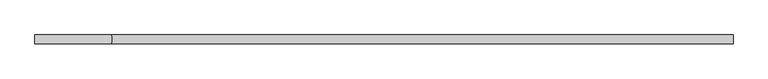
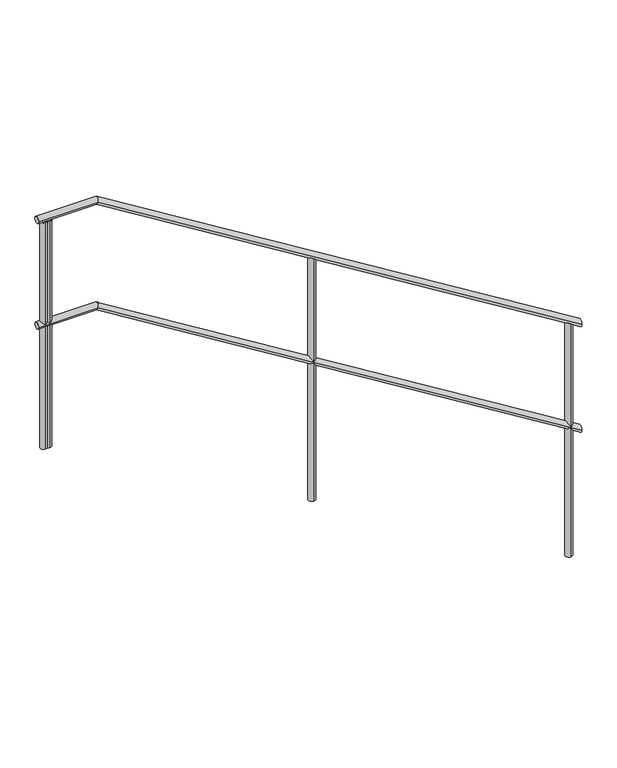
"""IFC4 building model written with IfcOpenShell, lengths in millimetres: railing geometry."""

from ifc_helpers import new_model, si_unit, point, frame, frame_2d, origin, place, context, project, spatial, circle_curve, ellipse_curve, trimmed, segment, composite_curve, outline, extrude, source, transform, mapped, element, save
from ifc_brep_helpers import plane_surface, cylinder_surface, advanced_brep


def railing_0facc66a(model_context):
    return source(origin(), model_context, "Body", "SolidModel", [
        advanced_brep(
        [(33992.1378478, 64692.0208589, -450.9609787), (33992.1378478, 64662.0208589, -450.9609787), (31827.8810623, 64692.0208589, 885.0), (31827.8810623, 64662.0208589, 885.0), (31562.1378478, 64692.0208589, 885.0), (31562.1378478, 64662.0208589, 885.0)],
        [
            (0, 1, ellipse_curve(frame((33992.1378478, 64677.0208589, -450.9609787), z_axis=(1.0, 0.0, 0.0), x_axis=(0.0, 0.0, -1.0)), 17.6276454, 15.0)),
            (1, 0, ellipse_curve(frame((33992.1378478, 64677.0208589, -450.9609787), z_axis=(1.0, 0.0, 0.0), x_axis=(0.0, 0.0, -1.0)), 17.6276454, 15.0)),
            (0, 2),
            (2, 3, ellipse_curve(frame((31827.8810623, 64677.0208589, 885.0), z_axis=(0.9620125025549408, 0.0, -0.2730053935877092), x_axis=(-0.2730053935877086, 0.0, -0.9620125025549411)), 15.5923129, 15.0)),
            (3, 1),
            (3, 2, ellipse_curve(frame((31827.8810623, 64677.0208589, 885.0), z_axis=(0.9620125025549408, 0.0, -0.2730053935877092), x_axis=(-0.2730053935877086, 0.0, -0.9620125025549411)), 15.5923129, 15.0)),
            (4, 5, circle_curve(frame((31562.1378478, 64677.0208589, 885.0), z_axis=(-1.0, 0.0, 0.0), x_axis=(0.0, -1.0, 0.0)), 15.0)),
            (5, 4, circle_curve(frame((31562.1378478, 64677.0208589, 885.0), z_axis=(-1.0, 0.0, 0.0), x_axis=(0.0, -1.0, 0.0)), 15.0)),
            (2, 4),
            (5, 3),
        ],
        [
            plane_surface(frame((33992.1378478, 64677.0208589, -433.3333333), z_axis=(1.0, 0.0, 0.0), x_axis=(0.0, -1.0, 0.0))),
            cylinder_surface(frame((33984.2588097, 64677.0208589, -446.097375), z_axis=(0.8509361101440399, 0.0, -0.5252692037926175), x_axis=(0.0, -1.0, 0.0)), 15.0),
            plane_surface(frame((31562.1378478, 64677.0208589, 900.0), z_axis=(-1.0, 0.0, 0.0), x_axis=(0.0, -1.0, 0.0))),
            cylinder_surface(frame((31832.1378478, 64677.0208589, 885.0), z_axis=(1.0, 0.0, 0.0), x_axis=(0.0, -1.0, 0.0)), 15.0),
        ],
        [
            (0, [[1, 2]]),
            (1, [[-1, 3, 4, 5]]),
            (1, [[-2, -5, 6, -3]]),
            (2, [[7, 8]]),
            (3, [[-4, 9, -8, 10]]),
            (3, [[-6, -10, -7, -9]]),
        ],
    ),
        advanced_brep(
        [(33992.1378478, 64692.0208589, 49.0390213), (33992.1378478, 64662.0208589, 49.0390213), (31827.8810623, 64692.0208589, 1385.0), (31827.8810623, 64662.0208589, 1385.0), (31562.1378478, 64692.0208589, 1385.0), (31562.1378478, 64662.0208589, 1385.0)],
        [
            (0, 1, ellipse_curve(frame((33992.1378478, 64677.0208589, 49.0390213), z_axis=(1.0, 0.0, 0.0), x_axis=(0.0, 0.0, -1.0)), 17.6276454, 15.0)),
            (1, 0, ellipse_curve(frame((33992.1378478, 64677.0208589, 49.0390213), z_axis=(1.0, 0.0, 0.0), x_axis=(0.0, 0.0, -1.0)), 17.6276454, 15.0)),
            (0, 2),
            (2, 3, ellipse_curve(frame((31827.8810623, 64677.0208589, 1385.0), z_axis=(0.9620125025549408, 0.0, -0.2730053935877092), x_axis=(-0.2730053935877086, 0.0, -0.9620125025549411)), 15.5923129, 15.0)),
            (3, 1),
            (3, 2, ellipse_curve(frame((31827.8810623, 64677.0208589, 1385.0), z_axis=(0.9620125025549408, 0.0, -0.2730053935877092), x_axis=(-0.2730053935877086, 0.0, -0.9620125025549411)), 15.5923129, 15.0)),
            (4, 5, circle_curve(frame((31562.1378478, 64677.0208589, 1385.0), z_axis=(-1.0, 0.0, 0.0), x_axis=(0.0, -1.0, 0.0)), 15.0)),
            (5, 4, circle_curve(frame((31562.1378478, 64677.0208589, 1385.0), z_axis=(-1.0, 0.0, 0.0), x_axis=(0.0, -1.0, 0.0)), 15.0)),
            (2, 4),
            (5, 3),
        ],
        [
            plane_surface(frame((33992.1378478, 64677.0208589, 66.6666667), z_axis=(1.0, 0.0, 0.0), x_axis=(0.0, -1.0, 0.0))),
            cylinder_surface(frame((33984.2588097, 64677.0208589, 53.902625), z_axis=(0.8509361101440399, 0.0, -0.5252692037926175), x_axis=(0.0, -1.0, 0.0)), 15.0),
            plane_surface(frame((31562.1378478, 64677.0208589, 1400.0), z_axis=(-1.0, 0.0, 0.0), x_axis=(0.0, -1.0, 0.0))),
            cylinder_surface(frame((31832.1378478, 64677.0208589, 1385.0), z_axis=(1.0, 0.0, 0.0), x_axis=(0.0, -1.0, 0.0)), 15.0),
        ],
        [
            (0, [[1, 2]]),
            (1, [[-1, 3, 4, 5]]),
            (1, [[-2, -5, 6, -3]]),
            (2, [[7, 8]]),
            (3, [[-4, 9, -8, 10]]),
            (3, [[-6, -10, -7, -9]]),
        ],
    ),
        extrude(outline(composite_curve([segment(trimmed(circle_curve(frame_2d((31592.1378478, 64677.0208589)), 15.0), [point((31592.1378478, 64692.0208589))], [point((31592.1378478, 64662.0208589))], False, "CARTESIAN"), True, "CONTINUOUS"), segment(trimmed(circle_curve(frame_2d((31592.1378478, 64677.0208589)), 15.0), [point((31592.1378478, 64662.0208589))], [point((31592.1378478, 64692.0208589))], False, "CARTESIAN"), True, "CONTINUOUS")], self_intersect=False)), frame((0.0, 0.0, 300.0), z_axis=(0.0, 0.0, 1.0), x_axis=(1.0, 0.0, 0.0)), (0.0, 0.0, 1.0), 1070.0),
        advanced_brep(
        [(32792.1378478, 64662.0208589, 777.4074074), (32792.1378478, 64692.0208589, 777.4074074), (32792.1378478, 64692.0208589, -366.6666667), (32792.1378478, 64662.0208589, -366.6666667)],
        [
            (0, 1, ellipse_curve(frame((32792.1378478, 64677.0208589, 777.4074074), z_axis=(-0.5252692037926167, 0.0, -0.8509361101440406), x_axis=(-0.8509361101440406, 0.0, 0.5252692037926162)), 17.6276454, 15.0)),
            (1, 2),
            (2, 3, circle_curve(frame((32792.1378478, 64677.0208589, -366.6666667), z_axis=(0.0, 0.0, 1.0), x_axis=(0.0, 1.0, 0.0)), 15.0)),
            (3, 0),
            (3, 2, circle_curve(frame((32792.1378478, 64677.0208589, -366.6666667), z_axis=(0.0, 0.0, 1.0), x_axis=(0.0, 1.0, 0.0)), 15.0)),
            (1, 0, ellipse_curve(frame((32792.1378478, 64677.0208589, 777.4074074), z_axis=(-0.5252692037926167, 0.0, -0.8509361101440406), x_axis=(-0.8509361101440406, 0.0, 0.5252692037926162)), 17.6276454, 15.0)),
        ],
        [
            cylinder_surface(frame((32792.1378478, 64677.0208589, -466.6666667), z_axis=(0.0, 0.0, 1.0), x_axis=(0.0, 1.0, 0.0)), 15.0),
            plane_surface(frame((32767.1378478, 64702.0208589, 792.8395062), z_axis=(0.5252692037926167, 0.0, 0.8509361101440406), x_axis=(0.0, -1.0, 0.0))),
            plane_surface(frame((32817.1378478, 64702.0208589, -366.6666667), z_axis=(0.0, 0.0, -1.0), x_axis=(0.0, -1.0, 0.0))),
        ],
        [
            (0, [[1, 2, 3, 4]]),
            (0, [[5, -2, 6, -4]]),
            (1, [[-6, -1]]),
            (2, [[-5, -3]]),
        ],
    ),
        extrude(outline(composite_curve([segment(trimmed(circle_curve(frame_2d((31612.1378478, 64677.0208589)), 15.0), [point((31612.1378478, 64692.0208589))], [point((31612.1378478, 64662.0208589))], False, "CARTESIAN"), True, "CONTINUOUS"), segment(trimmed(circle_curve(frame_2d((31612.1378478, 64677.0208589)), 15.0), [point((31612.1378478, 64662.0208589))], [point((31612.1378478, 64692.0208589))], False, "CARTESIAN"), True, "CONTINUOUS")], self_intersect=False)), frame((0.0, 0.0, 300.0), z_axis=(0.0, 0.0, 1.0), x_axis=(1.0, 0.0, 0.0)), (0.0, 0.0, 1.0), 1070.0),
        advanced_brep(
        [(33942.1378478, 64662.0208589, 67.5308642), (33942.1378478, 64692.0208589, 67.5308642), (33942.1378478, 64692.0208589, -1033.3333333), (33942.1378478, 64662.0208589, -1033.3333333)],
        [
            (0, 1, ellipse_curve(frame((33942.1378478, 64677.0208589, 67.5308642), z_axis=(-0.5252692037926167, 0.0, -0.8509361101440406), x_axis=(-0.8509361101440406, 0.0, 0.5252692037926162)), 17.6276454, 15.0)),
            (1, 2),
            (2, 3, circle_curve(frame((33942.1378478, 64677.0208589, -1033.3333333), z_axis=(0.0, 0.0, 1.0), x_axis=(0.0, 1.0, 0.0)), 15.0)),
            (3, 0),
            (3, 2, circle_curve(frame((33942.1378478, 64677.0208589, -1033.3333333), z_axis=(0.0, 0.0, 1.0), x_axis=(0.0, 1.0, 0.0)), 15.0)),
            (1, 0, ellipse_curve(frame((33942.1378478, 64677.0208589, 67.5308642), z_axis=(-0.5252692037926167, 0.0, -0.8509361101440406), x_axis=(-0.8509361101440406, 0.0, 0.5252692037926162)), 17.6276454, 15.0)),
        ],
        [
            cylinder_surface(frame((33942.1378478, 64677.0208589, -1133.3333333), z_axis=(0.0, 0.0, 1.0), x_axis=(0.0, 1.0, 0.0)), 15.0),
            plane_surface(frame((33917.1378478, 64702.0208589, 82.962963), z_axis=(0.5252692037926167, 0.0, 0.8509361101440406), x_axis=(0.0, -1.0, 0.0))),
            plane_surface(frame((33967.1378478, 64702.0208589, -1033.3333333), z_axis=(0.0, 0.0, -1.0), x_axis=(0.0, -1.0, 0.0))),
        ],
        [
            (0, [[1, 2, 3, 4]]),
            (0, [[5, -2, 6, -4]]),
            (1, [[-6, -1]]),
            (2, [[-5, -3]]),
        ],
    ),
    ])


if __name__ == "__main__":
    model = new_model("IFC4")
    model_context = context("Model", 3, world=origin())
    ifc_project = project(units=[si_unit("LENGTHUNIT", "METRE", prefix="MILLI")], contexts=[model_context])
    site = spatial("IfcSite", under=ifc_project)
    building = spatial("IfcBuilding", under=site)
    placement = place(None, origin())
    railing_shape = railing_0facc66a(model_context)
    element("IfcRailing", 1, at=placement, inside=building, context=model_context, shape_type="MappedRepresentation", body=[
        mapped(railing_shape, transform((0.0, 0.0, 0.0), x_axis=(1.0, 0.0, 0.0), y_axis=(0.0, 1.0, 0.0), z_axis=(0.0, 0.0, 1.0))),
    ])
    save(model, "model.ifc")
